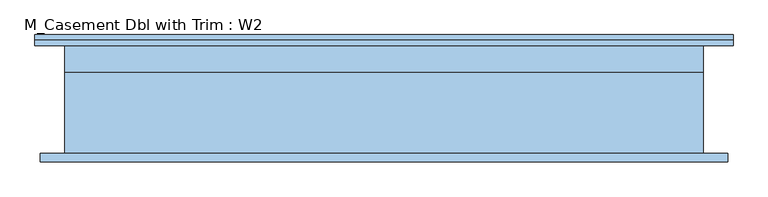
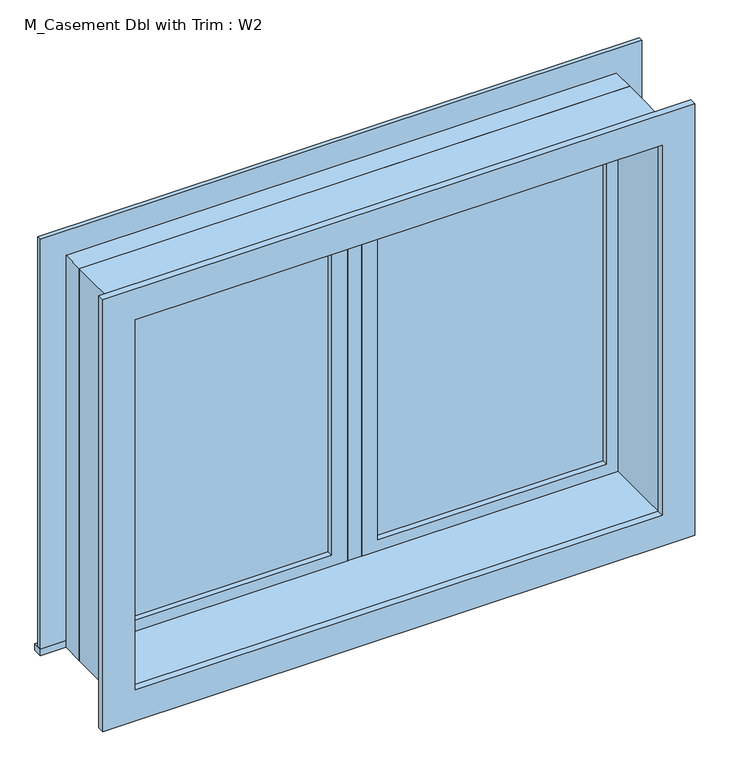
"""IFC4 building model written with IfcOpenShell, lengths in millimetres: window geometry, M_Casement Dbl with Trim : W2."""

from ifc_helpers import new_model, si_unit, frame, origin, place, context, project, spatial, polyline, outline, extrude, source, transform, mapped, element, save


def m_casement_dbl_with_trim_w2_d0a2a0c6(model_context):
    return source(origin(), model_context, "Body", "SweptSolid", [
        extrude(outline(polyline([(63.5, 111.175), (686.5, 111.175), (686.5, 98.475), (63.5, 98.475), (63.5, 111.175)])), frame((0.0, 0.0, 963.5), z_axis=(0.0, 0.0, 1.0), x_axis=(1.0, 0.0, 0.0)), (0.0, 0.0, 1.0), 1003.0),
        extrude(outline(polyline([(2010.95, 19.05), (919.05, 19.05), (919.05, 730.95), (2010.95, 730.95), (2010.95, 19.05)]), holes=[polyline([(1966.5, 63.5), (1966.5, 686.5), (963.5, 686.5), (963.5, 63.5), (1966.5, 63.5)])]), frame((0.0, 82.6, 0.0), z_axis=(0.0, 1.0, 0.0), x_axis=(0.0, 0.0, 1.0)), (0.0, 0.0, 1.0), 44.45),
        extrude(outline(polyline([(-819.95, 171.75), (819.95, 171.75), (819.95, 146.05), (-819.95, 146.05), (-819.95, 171.75)])), frame((0.0, 0.0, 900.0), z_axis=(0.0, 0.0, 1.0), x_axis=(1.0, 0.0, 0.0)), (0.0, 0.0, 1.0), 19.05),
        extrude(outline(polyline([(2010.95, -730.95), (2010.95, 730.95), (919.05, 730.95), (919.05, 819.95), (2099.95, 819.95), (2099.95, -819.95), (919.05, -819.95), (919.05, -730.95), (2010.95, -730.95)])), frame((0.0, 146.05, 0.0), z_axis=(0.0, 1.0, 0.0), x_axis=(0.0, 0.0, 1.0)), (0.0, 0.0, 1.0), 13.0),
        extrude(outline(polyline([(2087.25, 807.25), (2087.25, -807.25), (842.75, -807.25), (842.75, 807.25), (2087.25, 807.25)]), holes=[polyline([(1998.25, 718.25), (931.75, 718.25), (931.75, -718.25), (1998.25, -718.25), (1998.25, 718.25)])]), frame((0.0, -126.95, 0.0), z_axis=(0.0, 1.0, 0.0), x_axis=(0.0, 0.0, 1.0)), (0.0, 0.0, 1.0), 19.0),
        extrude(outline(polyline([(-63.5, 98.475), (-686.5, 98.475), (-686.5, 111.175), (-63.5, 111.175), (-63.5, 98.475)])), frame((0.0, 0.0, 963.5), z_axis=(0.0, 0.0, 1.0), x_axis=(1.0, 0.0, 0.0)), (0.0, 0.0, 1.0), 1003.0),
        extrude(outline(polyline([(2010.95, -730.95), (919.05, -730.95), (919.05, -19.05), (2010.95, -19.05), (2010.95, -730.95)]), holes=[polyline([(1966.5, -686.5), (1966.5, -63.5), (963.5, -63.5), (963.5, -686.5), (1966.5, -686.5)])]), frame((0.0, 82.6, 0.0), z_axis=(0.0, 1.0, 0.0), x_axis=(0.0, 0.0, 1.0)), (0.0, 0.0, 1.0), 44.45),
        extrude(outline(polyline([(2030.0, -750.0), (900.0, -750.0), (900.0, 750.0), (2030.0, 750.0), (2030.0, -750.0)]), holes=[polyline([(1998.25, -718.25), (1998.25, 718.25), (931.75, 718.25), (931.75, -718.25), (1998.25, -718.25)])]), frame((0.0, -107.95, 0.0), z_axis=(0.0, 1.0, 0.0), x_axis=(0.0, 0.0, 1.0)), (0.0, 0.0, 1.0), 190.55),
        extrude(outline(polyline([(2030.0, 750.0), (2030.0, -750.0), (900.0, -750.0), (900.0, 750.0), (2030.0, 750.0)]), holes=[polyline([(2010.95, 730.95), (919.05, 730.95), (919.05, -730.95), (2010.95, -730.95), (2010.95, 730.95)])]), frame((0.0, 82.6, 0.0), z_axis=(0.0, 1.0, 0.0), x_axis=(0.0, 0.0, 1.0)), (0.0, 0.0, 1.0), 63.45),
        extrude(outline(polyline([(19.05, 82.6), (-19.05, 82.6), (-19.05, 146.1), (19.05, 146.1), (19.05, 82.6)])), frame((0.0, 0.0, 919.05), z_axis=(0.0, 0.0, 1.0), x_axis=(1.0, 0.0, 0.0)), (0.0, 0.0, 1.0), 1091.9),
    ])


if __name__ == "__main__":
    model = new_model("IFC4")
    model_context = context("Model", 3, world=origin())
    ifc_project = project(units=[si_unit("LENGTHUNIT", "METRE", prefix="MILLI")], contexts=[model_context])
    site = spatial("IfcSite", under=ifc_project)
    building = spatial("IfcBuilding", under=site)
    placement = place(None, origin())
    m_casement_dbl_with_trim_w2_shape = m_casement_dbl_with_trim_w2_d0a2a0c6(model_context)
    element("IfcWindow", 1, ObjectType="M_Casement Dbl with Trim : W2", at=placement, inside=building, context=model_context, shape_type="MappedRepresentation", body=[
        mapped(m_casement_dbl_with_trim_w2_shape, transform((0.0, 0.0, 0.0), x_axis=(1.0, 0.0, 0.0), y_axis=(0.0, 1.0, 0.0), z_axis=(0.0, 0.0, 1.0))),
    ])
    save(model, "model.ifc")

# Revit data of these elements
# Type "M_Casement Dbl with Trim : W2"
#   Type Mark = "W2"
#   Construction Type Id = "GSP4R"
#   Analytic Construction = "1/8 in Pilkington single glazing"
#   Cost = 15000
#   Visual Light Transmittance = 0.9
#   Solar Heat Gain Coefficient = 0.78
#   Heat Transfer Coefficient (U) = 3.6886 W/(m²·K)
#   Height = 1130 mm
#   Default Sill Height = 900 mm
#   Trim Projection - Ext. = 13 mm
#   Trim Projection - Int. = 19 mm
#   Trim Width - Exterior = 89 mm
#   Trim Width - Interior = 89 mm
#   Width = 1500 mm
#   Window Inset = 19 mm
#   Glass Pane Material = Glass
#   Sash = wooden-3
#   Trim Exterior Material = wooden-3
#   Trim Interior Material = wooden-3
#   Wall Closure = (empty or 0)
# Element 1 (IfcWindow, "M_Casement Dbl with Trim : W2")
#   Materials on its faces: "wooden-3", "Glass"
# Materials
#   "Glass": class "Glass", colour RGB 140 218 255, transparency 0.75, Description = "Soda Lime Glass", Cost = 0
#   "wooden-3": class "Generic", colour RGB 120 120 120, transparency 0, Cost = 0
